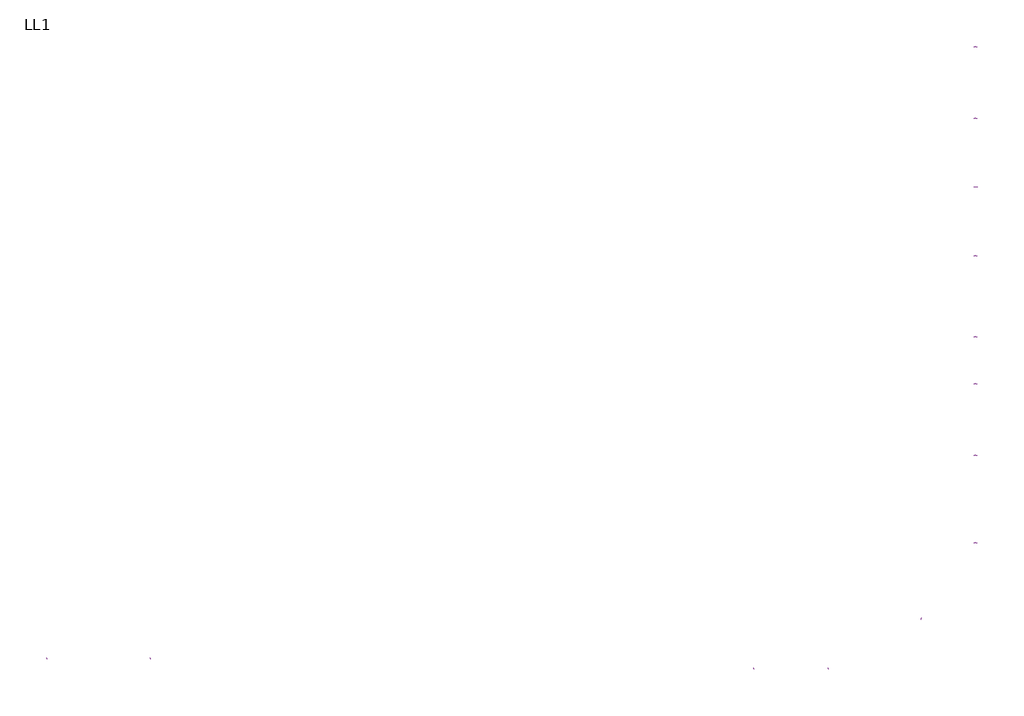
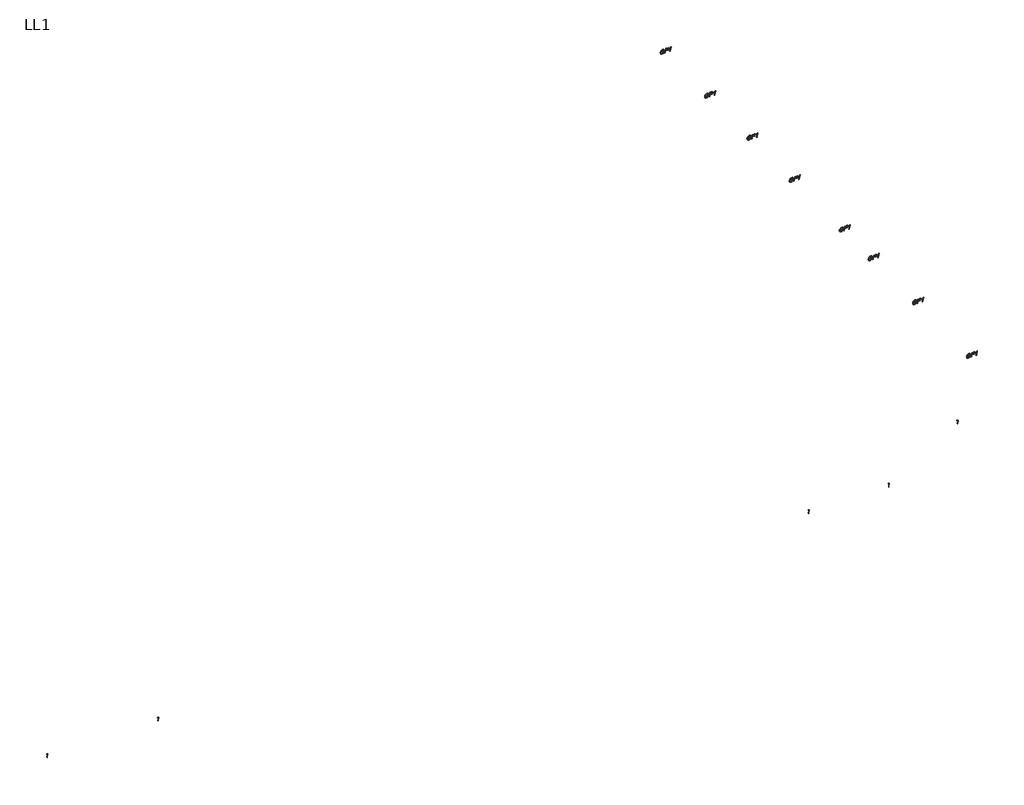
# One storey: 13 proxies.
"""IFC4 building model written with IfcOpenShell, lengths in millimetres."""

import ifcopenshell
import ifcopenshell.guid

model = None  # the IFC model being written
_history = None  # IfcOwnerHistory: only IFC2X3 demands one
_inside = {}  # id of a spatial element -> (the spatial element, [elements in it])
_under = {}  # id of a project, library or spatial element -> (it, [spatial elements below it])
_declared = {}  # id of a project -> (the project, [libraries it declares])
_typed = {}  # id of a type object -> (the type object, [elements of that type])
_made_of = {}  # id of a material, layer set ... -> (it, [elements and type objects made of it])


def new_model(schema):
    """Start an empty IFC model of exactly this schema.

    Asked for "IFC4X3", IfcOpenShell would pick the latest addendum, in which some entities
    have other attributes; the version numbers below select the first issue.
    IFC2X3 requires an IfcOwnerHistory on every rooted entity: one is made here for all.
    """
    global model, _history
    if schema == "IFC4X3":
        model = ifcopenshell.file(schema_version=(4, 3, 0, 0))
    else:
        model = ifcopenshell.file(schema=schema)
    _inside.clear()
    _under.clear()
    _declared.clear()
    _typed.clear()
    _made_of.clear()
    _history = None
    if model.schema == "IFC2X3":
        org = make("IfcOrganization", Name="unknown")
        user = make(
            "IfcPersonAndOrganization",
            ThePerson=make("IfcPerson", FamilyName="unknown"),
            TheOrganization=org,
        )
        app = make(
            "IfcApplication",
            ApplicationDeveloper=org,
            Version="unknown",
            ApplicationFullName="unknown",
            ApplicationIdentifier="unknown",
        )
        _history = make(
            "IfcOwnerHistory",
            OwningUser=user,
            OwningApplication=app,
            ChangeAction="ADDED",
            CreationDate=0,
        )
    return model


def make(cls, **values):
    """One entity of the class cls with the attributes given. An attribute that is None is left unset."""
    return model.create_entity(
        cls, **{name: value for name, value in values.items() if value is not None}
    )


def rooted(cls, **values):
    """An entity with a GlobalId (a new one), such as an element, a storey or a relation."""
    return make(cls, GlobalId=ifcopenshell.guid.new(), OwnerHistory=_history, **values)


def si_unit(unit_type, name, prefix=None):
    """IfcSIUnit, for example si_unit("LENGTHUNIT", "METRE", prefix="MILLI")."""
    return make("IfcSIUnit", UnitType=unit_type, Prefix=prefix, Name=name)


def assignment(units):
    """IfcUnitAssignment: the units of a project."""
    return None if units is None else make("IfcUnitAssignment", Units=units)


def point(xyz):
    """IfcCartesianPoint."""
    return None if xyz is None else make("IfcCartesianPoint", Coordinates=xyz)


def direction(xyz):
    """IfcDirection."""
    return None if xyz is None else make("IfcDirection", DirectionRatios=xyz)


def frame(location, z_axis=None, x_axis=None):
    """IfcAxis2Placement3D, a coordinate frame: its origin and axes. An axis left out is left unset."""
    return make(
        "IfcAxis2Placement3D",
        Location=point(location),
        Axis=direction(z_axis),
        RefDirection=direction(x_axis),
    )


def origin():
    """The frame at (0, 0, 0) with its axes left unset."""
    return frame((0.0, 0.0, 0.0))


def place(relative_to, where):
    """IfcLocalPlacement: puts the frame where relative to a parent placement (None: the world)."""
    return make(
        "IfcLocalPlacement", PlacementRelTo=relative_to, RelativePlacement=where
    )


def context(
    kind, dimensions, precision=None, world=None, true_north=None, identifier=None
):
    """IfcGeometricRepresentationContext, for example the 3D "Model" context."""
    return make(
        "IfcGeometricRepresentationContext",
        ContextIdentifier=identifier,
        ContextType=kind,
        CoordinateSpaceDimension=dimensions,
        Precision=precision,
        WorldCoordinateSystem=world,
        TrueNorth=true_north,
    )


def project(units=None, contexts=None):
    """IfcProject with its units and contexts."""
    return rooted(
        "IfcProject",
        Name="project",
        RepresentationContexts=contexts,
        UnitsInContext=assignment(units),
    )


def spatial(cls, under=None, at=None, **own):
    """A site, building, storey or space (cls), placed at a placement, below another one or the project."""
    s = rooted(cls, ObjectPlacement=at, **own)
    if under is not None:
        _under.setdefault(under.id(), (under, []))[1].append(s)
    return s


def polyline(points):
    """IfcPolyline through the points."""
    return make("IfcPolyline", Points=[point(p) for p in points])


def outline(outer, holes=None, kind="AREA"):
    """IfcArbitraryClosedProfileDef: a profile drawn as a closed curve; with holes, ...WithVoids."""
    if holes is None:
        return make("IfcArbitraryClosedProfileDef", ProfileType=kind, OuterCurve=outer)
    return make(
        "IfcArbitraryProfileDefWithVoids",
        ProfileType=kind,
        OuterCurve=outer,
        InnerCurves=holes,
    )


def extrude(swept, where, along, depth):
    """IfcExtrudedAreaSolid: the profile swept, set in the frame where, extruded along a direction by depth."""
    return make(
        "IfcExtrudedAreaSolid",
        SweptArea=swept,
        Position=where,
        ExtrudedDirection=direction(along),
        Depth=depth,
    )


def shape(context_of_items, identifier, shape_type, items):
    """IfcShapeRepresentation: the items that make up one representation, for example the "Body"."""
    return make(
        "IfcShapeRepresentation",
        ContextOfItems=context_of_items,
        RepresentationIdentifier=identifier,
        RepresentationType=shape_type,
        Items=items,
    )


def source(mapping_origin, context_of_items, identifier, shape_type, items):
    """IfcRepresentationMap: a shape defined once, which mapped items show again and again."""
    return make(
        "IfcRepresentationMap",
        MappingOrigin=mapping_origin,
        MappedRepresentation=shape(context_of_items, identifier, shape_type, items),
    )


def transform(
    local_origin,
    x_axis=None,
    y_axis=None,
    z_axis=None,
    scale=None,
    scale2=None,
    scale3=None,
    uniform=True,
):
    """IfcCartesianTransformationOperator3D, or its non-uniform kind. x_axis, y_axis, z_axis: its Axis1, 2, 3."""
    if uniform:
        return make(
            "IfcCartesianTransformationOperator3D",
            Axis1=direction(x_axis),
            Axis2=direction(y_axis),
            LocalOrigin=point(local_origin),
            Scale=scale,
            Axis3=direction(z_axis),
        )
    return make(
        "IfcCartesianTransformationOperator3DnonUniform",
        Axis1=direction(x_axis),
        Axis2=direction(y_axis),
        LocalOrigin=point(local_origin),
        Scale=scale,
        Axis3=direction(z_axis),
        Scale2=scale2,
        Scale3=scale3,
    )


def mapped(mapping_source, mapping_target):
    """IfcMappedItem: shows the shape of a source again, moved by a transform."""
    return make(
        "IfcMappedItem", MappingSource=mapping_source, MappingTarget=mapping_target
    )


def made_of(thing, what):
    """Note that an element or type object is made of a material, layer set ...; save() writes the relation."""
    if what is not None:
        _made_of.setdefault(what.id(), (what, []))[1].append(thing)
    return thing


def element(
    cls,
    number,
    at=None,
    inside=None,
    cuts=None,
    type_object=None,
    material=None,
    context=None,
    identifier="Body",
    shape_type=None,
    held_by="IfcProductDefinitionShape",
    body=None,
    shapes=None,
    **own,
):
    """One element of the class cls, such as IfcWall. Its Tag is "e" and its number.

    at: its placement. inside: the storey or other place that contains it. cuts: it is an
    opening in that element (IfcRelVoidsElement). A single representation is given by context,
    identifier, shape_type and body (its items); several are given by shapes. held_by: the class
    of the entity that holds the representations. save() writes the other relations.
    """
    e = rooted(cls, Tag="e%d" % number, ObjectPlacement=at, **own)
    if body is not None:
        shapes = [shape(context, identifier, shape_type, body)]
    if shapes is not None:
        e.Representation = make(held_by, Representations=shapes)
    if inside is not None:
        _inside.setdefault(inside.id(), (inside, []))[1].append(e)
    if cuts is not None:
        rooted(
            "IfcRelVoidsElement", RelatingBuildingElement=cuts, RelatedOpeningElement=e
        )
    if type_object is not None:
        _typed.setdefault(type_object.id(), (type_object, []))[1].append(e)
    return made_of(e, material)


def aggregate(whole, parts):
    """IfcRelAggregates: a whole, such as a stair, and the parts it consists of."""
    return rooted("IfcRelAggregates", RelatingObject=whole, RelatedObjects=parts)


def save(model, path):
    """Write the relations noted so far, then the file.

    IfcRelAggregates (storeys below a building ...), IfcRelContainedInSpatialStructure (elements
    in a storey), IfcRelDefinesByType, IfcRelAssociatesMaterial and IfcRelDeclares: one each for
    every whole, place, type object, material and project.
    """
    for whole, parts in _under.values():
        aggregate(whole, parts)
    for where, things in _inside.values():
        rooted(
            "IfcRelContainedInSpatialStructure",
            RelatedElements=things,
            RelatingStructure=where,
        )
    for kind, things in _typed.values():
        rooted("IfcRelDefinesByType", RelatedObjects=things, RelatingType=kind)
    for what, things in _made_of.values():
        rooted("IfcRelAssociatesMaterial", RelatedObjects=things, RelatingMaterial=what)
    for by, libraries in _declared.values():
        rooted("IfcRelDeclares", RelatingContext=by, RelatedDefinitions=libraries)
    model.write(path)


def proxy_2011_grid_3d_grid_8daef3c7(model_context):
    return source(origin(), model_context, "Body", "SweptSolid", [
        extrude(outline(polyline([(-101.6, 32359.573927), (-101.6, 32385.4006614), (101.4447294, 32427.5859799), (101.4447294, 32412.7641112), (88.0108618, 32402.0071029), (67.0173455, 32374.5692958), (47.5109731, 32337.8120529), (25.3029559, 32333.152335), (36.729179, 32366.4271823), (51.3775476, 32391.299666), (-101.6, 32359.573927)])), frame((0.0, -3.175, 0.0), z_axis=(0.0, 1.0, 0.0), x_axis=(0.0, 0.0, 1.0)), (0.0, 0.0, 1.0), 3.175),
    ])


def proxy_2011_grid_3d_grid_89aafc61(model_context):
    return source(origin(), model_context, "Body", "SweptSolid", [
        extrude(outline(polyline([(-101.6, 29940.1966257), (-101.6, 29966.0233601), (101.4447294, 30008.2086786), (101.4447294, 29993.38681), (88.0108618, 29982.6298016), (67.0173455, 29955.1919945), (47.5109731, 29918.4347517), (25.3029559, 29913.7750337), (36.729179, 29947.0498811), (51.3775476, 29971.9223647), (-101.6, 29940.1966257)])), frame((0.0, -3.175, 0.0), z_axis=(0.0, 1.0, 0.0), x_axis=(0.0, 0.0, 1.0)), (0.0, 0.0, 1.0), 3.175),
    ])


def proxy_2011_grid_3d_grid_895aad00(model_context):
    return source(origin(), model_context, "Body", "SweptSolid", [
        extrude(outline(polyline([(-22.2856526, 47336.5225939), (-22.2856526, 47396.9997838), (-65.3632575, 47388.324777), (-78.2642318, 47358.8049683), (-82.5645566, 47331.3175898), (-78.6484107, 47307.5728571), (-66.899973, 47289.5784145), (-47.5051365, 47278.2389414), (-20.6497942, 47274.459117), (8.448657, 47277.3280657), (34.2753914, 47285.9349117), (55.4114257, 47299.3377971), (70.4377767, 47316.5948641), (79.4164087, 47336.510201), (82.409286, 47357.8878962), (79.5465338, 47377.2269648), (70.9582771, 47392.7118519), (56.9915162, 47403.9583785), (37.9932514, 47410.5823658), (41.1658253, 47435.9629569), (60.4119475, 47430.7393636), (75.617995, 47423.0000183), (87.4841649, 47412.0261347), (96.7106543, 47397.0989267), (102.640641, 47379.0920913), (104.6173033, 47358.8793255), (101.0419612, 47330.6297857), (90.315935, 47305.069498), (72.1170101, 47282.9358379), (46.1229721, 47264.9661811), (14.5831261, 47253.0504396), (-20.2532224, 47249.0785258), (-52.387926, 47253.5895294), (-78.1031246, 47267.1225399), (-89.7710087, 47279.2303707), (-98.1052116, 47294.089418), (-103.1057333, 47311.6996817), (-104.7725739, 47332.0611618), (-103.1243226, 47352.5713564), (-98.1795688, 47373.4533369), (-81.1765555, 47410.929366), (-0.0776353, 47427.3375217), (-0.0776353, 47341.4301691), (-22.2856526, 47336.5225939)])), frame((0.0, -3.175, 0.0), z_axis=(0.0, 1.0, 0.0), x_axis=(0.0, 0.0, 1.0)), (0.0, 0.0, 1.0), 3.175),
        extrude(outline(polyline([(-101.6, 47455.2958291), (-101.6, 47481.072992), (-9.595357, 47499.6622922), (-9.595357, 47605.4973745), (12.6126603, 47611.8425223), (12.6126603, 47504.1732957), (79.2367121, 47517.6567348), (79.2367121, 47618.5842419), (101.4447294, 47624.9293897), (101.4447294, 47496.3410039), (-101.6, 47455.2958291)])), frame((0.0, -3.175, 0.0), z_axis=(0.0, 1.0, 0.0), x_axis=(0.0, 0.0, 1.0)), (0.0, 0.0, 1.0), 3.175),
        extrude(outline(polyline([(-101.6, 47683.7211497), (-101.6, 47709.547884), (101.4447294, 47751.7332026), (101.4447294, 47736.9113339), (88.0108618, 47726.1543255), (67.0173455, 47698.7165185), (47.5109731, 47661.9592756), (25.3029559, 47657.2995577), (36.729179, 47690.574405), (51.3775476, 47715.4468886), (-101.6, 47683.7211497)])), frame((0.0, -3.175, 0.0), z_axis=(0.0, 1.0, 0.0), x_axis=(0.0, 0.0, 1.0)), (0.0, 0.0, 1.0), 3.175),
    ])


model = new_model("IFC4")

# Units and contexts
model_context = context("Model", 3, world=origin())
ifc_project = project(units=[si_unit("LENGTHUNIT", "METRE", prefix="MILLI")], contexts=[model_context])

# Site, building, storey
site = spatial("IfcSite", under=ifc_project)
building = spatial("IfcBuilding", under=site)
storey = spatial("IfcBuildingStorey", under=building, Name="LL1", Elevation=-3048.0)

# Proxies
placement = place(None, origin())
proxy_2011_grid_3d_grid_shape = proxy_2011_grid_3d_grid_8daef3c7(model_context)
element("IfcBuildingElementProxy", 1, Name="2011_Grid_3D : Grid", ObjectType="2011_Grid_3D : Grid", at=placement, inside=storey, context=model_context, shape_type="MappedRepresentation", body=[
    mapped(proxy_2011_grid_3d_grid_shape, transform((-7263.9497761, 15187.8351025, 0.0), x_axis=(0.0, -1.0, 0.0), y_axis=(1.0, 0.0, 0.0), z_axis=(0.0, 0.0, 1.0))),
])
element("IfcBuildingElementProxy", 2, Name="2011_Grid_3D : Grid", ObjectType="2011_Grid_3D : Grid", at=placement, inside=storey, context=model_context, shape_type="MappedRepresentation", body=[
    mapped(proxy_2011_grid_3d_grid_shape, transform((-2194.9109081, 15187.8351025, 0.0), x_axis=(0.0, -1.0, 0.0), y_axis=(1.0, 0.0, 0.0), z_axis=(0.0, 0.0, 1.0))),
])
element("IfcBuildingElementProxy", 3, Name="2011_Grid_3D : Grid", ObjectType="2011_Grid_3D : Grid", at=placement, inside=storey, context=model_context, shape_type="MappedRepresentation", body=[
    mapped(proxy_2011_grid_3d_grid_shape, transform((27257.8956172, 14700.6077512, 0.0), x_axis=(0.0, -1.0, 0.0), y_axis=(1.0, 0.0, 0.0), z_axis=(0.0, 0.0, 1.0))),
])
element("IfcBuildingElementProxy", 4, Name="2011_Grid_3D : Grid", ObjectType="2011_Grid_3D : Grid", at=placement, inside=storey, context=model_context, shape_type="MappedRepresentation", body=[
    mapped(proxy_2011_grid_3d_grid_shape, transform((30915.4956172, 14700.6077512, 0.0), x_axis=(0.0, -1.0, 0.0), y_axis=(1.0, 0.0, 0.0), z_axis=(0.0, 0.0, 1.0))),
])
proxy_2011_grid_3d_grid_2_shape = proxy_2011_grid_3d_grid_89aafc61(model_context)
element("IfcBuildingElementProxy", 5, Name="2011_Grid_3D : Grid", ObjectType="2011_Grid_3D : Grid", at=placement, inside=storey, context=model_context, shape_type="MappedRepresentation", body=[
    mapped(proxy_2011_grid_3d_grid_2_shape, transform((35447.8890919, 14700.6077512, 0.0), x_axis=(0.0, -1.0, 0.0), y_axis=(1.0, 0.0, 0.0), z_axis=(0.0, 0.0, 1.0))),
])
proxy_2011_grid_3d_grid_3_shape = proxy_2011_grid_3d_grid_895aad00(model_context)
element("IfcBuildingElementProxy", 6, Name="2011_Grid_3D : Grid", ObjectType="2011_Grid_3D : Grid", at=placement, inside=storey, context=model_context, shape_type="MappedRepresentation", body=[
    mapped(proxy_2011_grid_3d_grid_3_shape, transform((-9245.1497761, 12690.6740284, 0.0), x_axis=(1.0, 0.0, 0.0), y_axis=(0.0, 1.0, 0.0), z_axis=(0.0, 0.0, 1.0))),
])
element("IfcBuildingElementProxy", 7, Name="2011_Grid_3D : Grid", ObjectType="2011_Grid_3D : Grid", at=placement, inside=storey, context=model_context, shape_type="MappedRepresentation", body=[
    mapped(proxy_2011_grid_3d_grid_3_shape, transform((-9245.1497761, 9185.4740284, 0.0), x_axis=(1.0, 0.0, 0.0), y_axis=(0.0, 1.0, 0.0), z_axis=(0.0, 0.0, 1.0))),
])
element("IfcBuildingElementProxy", 8, Name="2011_Grid_3D : Grid", ObjectType="2011_Grid_3D : Grid", at=placement, inside=storey, context=model_context, shape_type="MappedRepresentation", body=[
    mapped(proxy_2011_grid_3d_grid_3_shape, transform((-9245.1497761, 5832.6740284, 0.0), x_axis=(1.0, 0.0, 0.0), y_axis=(0.0, 1.0, 0.0), z_axis=(0.0, 0.0, 1.0))),
])
element("IfcBuildingElementProxy", 9, Name="2011_Grid_3D : Grid", ObjectType="2011_Grid_3D : Grid", at=placement, inside=storey, context=model_context, shape_type="MappedRepresentation", body=[
    mapped(proxy_2011_grid_3d_grid_3_shape, transform((-9245.1497761, 2479.8740284, 0.0), x_axis=(1.0, 0.0, 0.0), y_axis=(0.0, 1.0, 0.0), z_axis=(0.0, 0.0, 1.0))),
])
element("IfcBuildingElementProxy", 10, Name="2011_Grid_3D : Grid", ObjectType="2011_Grid_3D : Grid", at=placement, inside=storey, context=model_context, shape_type="MappedRepresentation", body=[
    mapped(proxy_2011_grid_3d_grid_3_shape, transform((-9245.1497761, -1482.5259716, 0.0), x_axis=(1.0, 0.0, 0.0), y_axis=(0.0, 1.0, 0.0), z_axis=(0.0, 0.0, 1.0))),
])
element("IfcBuildingElementProxy", 11, Name="2011_Grid_3D : Grid", ObjectType="2011_Grid_3D : Grid", at=placement, inside=storey, context=model_context, shape_type="MappedRepresentation", body=[
    mapped(proxy_2011_grid_3d_grid_3_shape, transform((-9245.1497761, -3768.5259716, 0.0), x_axis=(1.0, 0.0, 0.0), y_axis=(0.0, 1.0, 0.0), z_axis=(0.0, 0.0, 1.0))),
])
element("IfcBuildingElementProxy", 12, Name="2011_Grid_3D : Grid", ObjectType="2011_Grid_3D : Grid", at=placement, inside=storey, context=model_context, shape_type="MappedRepresentation", body=[
    mapped(proxy_2011_grid_3d_grid_3_shape, transform((-9245.1497761, -7273.7259716, 0.0), x_axis=(1.0, 0.0, 0.0), y_axis=(0.0, 1.0, 0.0), z_axis=(0.0, 0.0, 1.0))),
])
element("IfcBuildingElementProxy", 13, Name="2011_Grid_3D : Grid", ObjectType="2011_Grid_3D : Grid", at=placement, inside=storey, context=model_context, shape_type="MappedRepresentation", body=[
    mapped(proxy_2011_grid_3d_grid_3_shape, transform((-9245.1497761, -11540.9259716, 0.0), x_axis=(1.0, 0.0, 0.0), y_axis=(0.0, 1.0, 0.0), z_axis=(0.0, 0.0, 1.0))),
])

save(model, "model.ifc")

# Revit data of these elements
# Project information
#   TBC Electrician = "ELECTRICIAN HERE"
#   TBC Fire Protection = "FP HERE"
#   TBC Plumber = "PLUMBER HERE"
#   TBC HVAC = "HVAC HERE"
#   TBC Other Company 1 = "MISC COMPANY 1"
#   TBC Other Company 2 = "MISC COMPANY 2"
#   TBC COORDINATOR = "NAME OF VCC"
#   Project Issue Date = "Issue Date"
#   Project Status = "Project Status"
#   Client Name = "Owner"
#   Project Address = "Street\nCity, ST"
#   Project Name = "Project Name"
#   Project Number = "XX-XXX"
#   TBC Template Version = "2008-09-18"
# Grids (mm)
#   "8": line (37826.148, 12690.674) -> (-9245.15, 12690.674)
#   "9": line (37826.148, 9185.474) -> (-9245.15, 9185.474)
#   "10": line (37826.148, 5832.674) -> (-9245.15, 5832.674)
#   "11": line (37826.148, 2479.874) -> (-9245.15, 2479.874)
#   "12": line (37826.148, -1482.526) -> (-9245.15, -1482.526)
#   "13": line (37826.148, -3768.526) -> (-9245.15, -3768.526)
#   "14": line (37826.148, -7273.726) -> (-9245.15, -7273.726)
#   "15": line (37826.148, -11540.926) -> (-9245.15, -11540.926)
#   "3": line (-7263.95, -16949.542) -> (-7263.95, 15187.835)
#   "4": line (-2194.911, -16949.542) -> (-2194.911, 15187.835)
#   "5": line (3901.089, -16949.542) -> (3901.089, 15187.835)
#   "6": line (27257.896, -16949.542) -> (27257.896, 15187.835)
#   "7": line (30915.496, -16949.542) -> (30915.496, 15187.835)
#   "16": line (35447.889, -16949.542) -> (35447.889, 15187.835)
# Type "2011_Grid_3D : Grid"
#   Workplane [instance default] = "LEVEL"
#   Grid [instance default] = "S"
#   t [instance default] = 12' - 6"
#   built-in parameter 1001306 [instance default] = 50 (stored number, unit not read)
#   d [instance default] = 2
#   Symbol At End 2 [instance default] = yes
#   Symbol At End 1 [instance default] = yes
#   Robust [instance default] = yes
#   No of grid markers [instance default] = 3
#   Grid Height Visible = yes
#   Height = 0
#   Assembly Code = ""
# Element 1 (IfcBuildingElementProxy, "2011_Grid_3D : Grid")
#   Workplane = "1"
#   Grid = "1"
#   t = 13' - 2.15638"
#   built-in parameter 1001306 = 105.438 (stored number, unit not read)
#   d = 4
#   Symbol At End 2 = yes
#   Symbol At End 1 = yes
#   Robust = no
#   No of grid markers = 5
#   Phase Created = 02 - TEMP
#   Materials on its faces: "Letter"
# Element 2 (IfcBuildingElementProxy, "2011_Grid_3D : Grid")
#   Workplane = "1"
#   Grid = "2"
#   t = 13' - 2.15638"
#   built-in parameter 1001306 = 105.438 (stored number, unit not read)
#   d = 4
#   Symbol At End 2 = yes
#   Symbol At End 1 = yes
#   Robust = no
#   No of grid markers = 5
#   Phase Created = 02 - TEMP
#   Materials on its faces: "Letter"
# Element 3 (IfcBuildingElementProxy, "2011_Grid_3D : Grid")
#   Workplane = "1"
#   Grid = "3"
#   t = 13' - 2.15638"
#   built-in parameter 1001306 = 105.438 (stored number, unit not read)
#   d = 4
#   Symbol At End 2 = yes
#   Symbol At End 1 = yes
#   Robust = no
#   No of grid markers = 5
#   Phase Created = 02 - TEMP
#   Materials on its faces: "Letter"
# Element 4 (IfcBuildingElementProxy, "2011_Grid_3D : Grid")
#   Workplane = "1"
#   Grid = "4"
#   t = 13' - 2.15638"
#   built-in parameter 1001306 = 105.438 (stored number, unit not read)
#   d = 4
#   Symbol At End 2 = yes
#   Symbol At End 1 = yes
#   Robust = no
#   No of grid markers = 5
#   Phase Created = 02 - TEMP
#   Materials on its faces: "Letter"
# Element 5 (IfcBuildingElementProxy, "2011_Grid_3D : Grid")
#   Workplane = "1"
#   Grid = "5"
#   t = 12' - 2 1/4"
#   built-in parameter 1001306 = 97.5 (stored number, unit not read)
#   d = 4
#   Symbol At End 2 = yes
#   Symbol At End 1 = yes
#   Robust = no
#   No of grid markers = 5
#   Phase Created = 02 - TEMP
#   Materials on its faces: "Letter"
# Element 6 (IfcBuildingElementProxy, "2011_Grid_3D : Grid")
#   Workplane = "GF1"
#   Grid = "A"
#   t = 11' - 0.37148"
#   built-in parameter 1001306 = 154.433 (stored number, unit not read)
#   d = 7
#   Symbol At End 2 = yes
#   Symbol At End 1 = yes
#   Robust = no
#   No of grid markers = 8
#   Phase Created = 02 - TEMP
#   Materials on its faces: "Letter"
# Element 7 (IfcBuildingElementProxy, "2011_Grid_3D : Grid")
#   Workplane = "GF1"
#   Grid = "B"
#   t = 11' - 0.37148"
#   built-in parameter 1001306 = 154.433 (stored number, unit not read)
#   d = 7
#   Symbol At End 2 = yes
#   Symbol At End 1 = yes
#   Robust = no
#   No of grid markers = 8
#   Phase Created = 02 - TEMP
#   Materials on its faces: "Letter"
# Element 8 (IfcBuildingElementProxy, "2011_Grid_3D : Grid")
#   Workplane = "GF1"
#   Grid = "C"
#   t = 11' - 0.37148"
#   built-in parameter 1001306 = 154.433 (stored number, unit not read)
#   d = 7
#   Symbol At End 2 = yes
#   Symbol At End 1 = yes
#   Robust = no
#   No of grid markers = 8
#   Phase Created = 02 - TEMP
#   Materials on its faces: "Letter"
# Element 9 (IfcBuildingElementProxy, "2011_Grid_3D : Grid")
#   Workplane = "GF1"
#   Grid = "D"
#   t = 11' - 0.37148"
#   built-in parameter 1001306 = 154.433 (stored number, unit not read)
#   d = 7
#   Symbol At End 2 = yes
#   Symbol At End 1 = yes
#   Robust = no
#   No of grid markers = 8
#   Phase Created = 02 - TEMP
#   Materials on its faces: "Letter"
# Element 10 (IfcBuildingElementProxy, "2011_Grid_3D : Grid")
#   Workplane = "GF1"
#   Grid = "E"
#   t = 11' - 0.37148"
#   built-in parameter 1001306 = 154.433 (stored number, unit not read)
#   d = 7
#   Symbol At End 2 = yes
#   Symbol At End 1 = yes
#   Robust = no
#   No of grid markers = 8
#   Phase Created = 02 - TEMP
#   Materials on its faces: "Letter"
# Element 11 (IfcBuildingElementProxy, "2011_Grid_3D : Grid")
#   Workplane = "GF1"
#   Grid = "F"
#   t = 11' - 0.37148"
#   built-in parameter 1001306 = 154.433 (stored number, unit not read)
#   d = 7
#   Symbol At End 2 = yes
#   Symbol At End 1 = yes
#   Robust = no
#   No of grid markers = 8
#   Phase Created = 02 - TEMP
#   Materials on its faces: "Letter"
# Element 12 (IfcBuildingElementProxy, "2011_Grid_3D : Grid")
#   Workplane = "GF1"
#   Grid = "G"
#   t = 11' - 0.37148"
#   built-in parameter 1001306 = 154.433 (stored number, unit not read)
#   d = 7
#   Symbol At End 2 = yes
#   Symbol At End 1 = yes
#   Robust = no
#   No of grid markers = 8
#   Phase Created = 02 - TEMP
#   Materials on its faces: "Letter"
# Element 13 (IfcBuildingElementProxy, "2011_Grid_3D : Grid")
#   Workplane = "GF1"
#   Grid = "H"
#   t = 11' - 0.37148"
#   built-in parameter 1001306 = 154.433 (stored number, unit not read)
#   d = 7
#   Symbol At End 2 = yes
#   Symbol At End 1 = yes
#   Robust = no
#   No of grid markers = 8
#   Phase Created = 02 - TEMP
#   Materials on its faces: "Letter"
# Materials
#   "Letter": class "Unassigned", colour RGB 178 187 30, transparency 0, Comments = "Rendering appearance not upgraded "
